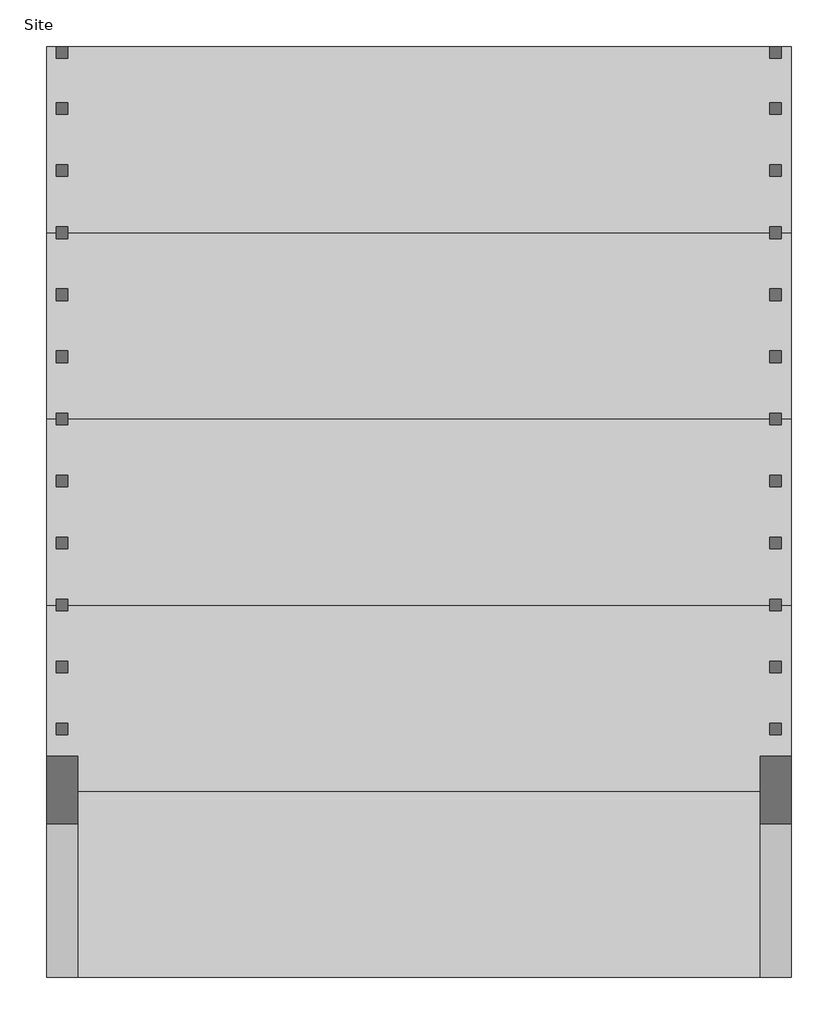
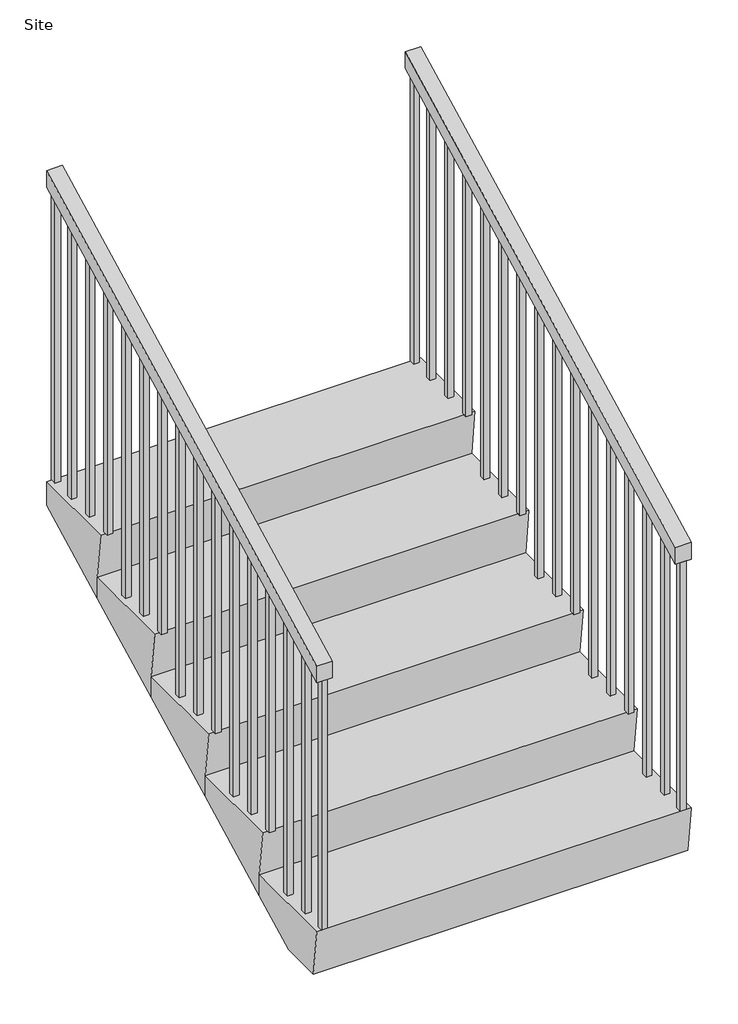
# One storey: 2 railings, 1 stair flight.
"""IFC4 building model written with IfcOpenShell, lengths in millimetres."""

from ifc_helpers import new_model, si_unit, frame, origin, place, context, project, spatial, polyline, outline, extrude, faceted_brep, element, save

model = new_model("IFC4")

# Units and contexts
model_context = context("Model", 3, world=origin())
ifc_project = project(units=[si_unit("LENGTHUNIT", "METRE", prefix="MILLI")], contexts=[model_context])

# Site, building, storey
site = spatial("IfcSite", under=ifc_project)
building = spatial("IfcBuilding", under=site)
storey = spatial("IfcBuildingStorey", under=building, Name="Site", Elevation=-939.8)

# Railings
placement = place(None, origin())
element("IfcRailing", 1, ObjectType="Handrail - Rectangular", at=placement, inside=storey, context=model_context, shape_type="SweptSolid", body=[
    extrude(outline(polyline([(-5687.1111242, 74.1181862), (-5687.1111242, 131.2333333), (-4163.1111242, 914.4), (-4163.1111242, 857.2848529), (-5687.1111242, 74.1181862)])), frame((-477.3803068, 0.0, 0.0), z_axis=(1.0, 0.0, 0.0), x_axis=(0.0, 1.0, 0.0)), (0.0, 0.0, 1.0), 50.8),
    extrude(outline(polyline([(-4274.2361242, 800.1789501), (-4255.1861242, 809.9685334), (-4255.1861242, -156.6333333), (-4274.2361242, -156.6333333), (-4274.2361242, 800.1789501)])), frame((-461.5053068, 0.0, 0.0), z_axis=(1.0, 0.0, 0.0), x_axis=(0.0, 1.0, 0.0)), (0.0, 0.0, 1.0), 19.05),
    extrude(outline(polyline([(-4375.8361242, 747.967839), (-4356.7861242, 757.7574223), (-4356.7861242, -156.6333333), (-4375.8361242, -156.6333333), (-4375.8361242, 747.967839)])), frame((-461.5053068, 0.0, 0.0), z_axis=(1.0, 0.0, 0.0), x_axis=(0.0, 1.0, 0.0)), (0.0, 0.0, 1.0), 19.05),
    extrude(outline(polyline([(-4477.4361242, 695.7567279), (-4458.3861242, 705.5463112), (-4458.3861242, -156.6333333), (-4477.4361242, -156.6333333), (-4477.4361242, 695.7567279)])), frame((-461.5053068, 0.0, 0.0), z_axis=(1.0, 0.0, 0.0), x_axis=(0.0, 1.0, 0.0)), (0.0, 0.0, 1.0), 19.05),
    extrude(outline(polyline([(-4579.0361242, 643.5456168), (-4559.9861242, 653.3352001), (-4559.9861242, -313.2666667), (-4579.0361242, -313.2666667), (-4579.0361242, 643.5456168)])), frame((-461.5053068, 0.0, 0.0), z_axis=(1.0, 0.0, 0.0), x_axis=(0.0, 1.0, 0.0)), (0.0, 0.0, 1.0), 19.05),
    extrude(outline(polyline([(-4680.6361242, 591.3345057), (-4661.5861242, 601.124089), (-4661.5861242, -313.2666667), (-4680.6361242, -313.2666667), (-4680.6361242, 591.3345057)])), frame((-461.5053068, 0.0, 0.0), z_axis=(1.0, 0.0, 0.0), x_axis=(0.0, 1.0, 0.0)), (0.0, 0.0, 1.0), 19.05),
    extrude(outline(polyline([(-4782.2361242, 539.1233945), (-4763.1861242, 548.9129779), (-4763.1861242, -313.2666667), (-4782.2361242, -313.2666667), (-4782.2361242, 539.1233945)])), frame((-461.5053068, 0.0, 0.0), z_axis=(1.0, 0.0, 0.0), x_axis=(0.0, 1.0, 0.0)), (0.0, 0.0, 1.0), 19.05),
    extrude(outline(polyline([(-4883.8361242, 486.9122834), (-4864.7861242, 496.7018668), (-4864.7861242, -469.9), (-4883.8361242, -469.9), (-4883.8361242, 486.9122834)])), frame((-461.5053068, 0.0, 0.0), z_axis=(1.0, 0.0, 0.0), x_axis=(0.0, 1.0, 0.0)), (0.0, 0.0, 1.0), 19.05),
    extrude(outline(polyline([(-4985.4361242, 434.7011723), (-4966.3861242, 444.4907557), (-4966.3861242, -469.9), (-4985.4361242, -469.9), (-4985.4361242, 434.7011723)])), frame((-461.5053068, 0.0, 0.0), z_axis=(1.0, 0.0, 0.0), x_axis=(0.0, 1.0, 0.0)), (0.0, 0.0, 1.0), 19.05),
    extrude(outline(polyline([(-5087.0361242, 382.4900612), (-5067.9861242, 392.2796445), (-5067.9861242, -469.9), (-5087.0361242, -469.9), (-5087.0361242, 382.4900612)])), frame((-461.5053068, 0.0, 0.0), z_axis=(1.0, 0.0, 0.0), x_axis=(0.0, 1.0, 0.0)), (0.0, 0.0, 1.0), 19.05),
    extrude(outline(polyline([(-5188.6361242, 330.2789501), (-5169.5861242, 340.0685334), (-5169.5861242, -626.5333333), (-5188.6361242, -626.5333333), (-5188.6361242, 330.2789501)])), frame((-461.5053068, 0.0, 0.0), z_axis=(1.0, 0.0, 0.0), x_axis=(0.0, 1.0, 0.0)), (0.0, 0.0, 1.0), 19.05),
    extrude(outline(polyline([(-5290.2361242, 278.067839), (-5271.1861242, 287.8574223), (-5271.1861242, -626.5333333), (-5290.2361242, -626.5333333), (-5290.2361242, 278.067839)])), frame((-461.5053068, 0.0, 0.0), z_axis=(1.0, 0.0, 0.0), x_axis=(0.0, 1.0, 0.0)), (0.0, 0.0, 1.0), 19.05),
    extrude(outline(polyline([(-5391.8361242, 225.8567279), (-5372.7861242, 235.6463112), (-5372.7861242, -626.5333333), (-5391.8361242, -626.5333333), (-5391.8361242, 225.8567279)])), frame((-461.5053068, 0.0, 0.0), z_axis=(1.0, 0.0, 0.0), x_axis=(0.0, 1.0, 0.0)), (0.0, 0.0, 1.0), 19.05),
    extrude(outline(polyline([(-5493.4361242, 173.6456168), (-5474.3861242, 183.4352001), (-5474.3861242, -783.1666667), (-5493.4361242, -783.1666667), (-5493.4361242, 173.6456168)])), frame((-461.5053068, 0.0, 0.0), z_axis=(1.0, 0.0, 0.0), x_axis=(0.0, 1.0, 0.0)), (0.0, 0.0, 1.0), 19.05),
    extrude(outline(polyline([(-5595.0361242, 121.4345057), (-5575.9861242, 131.224089), (-5575.9861242, -783.1666667), (-5595.0361242, -783.1666667), (-5595.0361242, 121.4345057)])), frame((-461.5053068, 0.0, 0.0), z_axis=(1.0, 0.0, 0.0), x_axis=(0.0, 1.0, 0.0)), (0.0, 0.0, 1.0), 19.05),
    extrude(outline(polyline([(-4182.1611242, 847.4952695), (-4163.1111242, 857.2848529), (-4163.1111242, -156.6333333), (-4182.1611242, -156.6333333), (-4182.1611242, 847.4952695)])), frame((-461.5053068, 0.0, 0.0), z_axis=(1.0, 0.0, 0.0), x_axis=(0.0, 1.0, 0.0)), (0.0, 0.0, 1.0), 19.05),
    extrude(outline(polyline([(-5687.1111242, 74.1181862), (-5668.0611242, 83.9077695), (-5668.0611242, -783.1666667), (-5687.1111242, -783.1666667), (-5687.1111242, 74.1181862)])), frame((-461.5053068, 0.0, 0.0), z_axis=(1.0, 0.0, 0.0), x_axis=(0.0, 1.0, 0.0)), (0.0, 0.0, 1.0), 19.05),
])
element("IfcRailing", 2, ObjectType="Handrail - Rectangular", at=placement, inside=storey, context=model_context, shape_type="SweptSolid", body=[
    extrude(outline(polyline([(-5687.1111242, 74.1181862), (-5687.1111242, 131.2333333), (-4163.1111242, 914.4), (-4163.1111242, 857.2848529), (-5687.1111242, 74.1181862)])), frame((-1645.7803068, 0.0, 0.0), z_axis=(1.0, 0.0, 0.0), x_axis=(0.0, 1.0, 0.0)), (0.0, 0.0, 1.0), 50.8),
    extrude(outline(polyline([(-4255.1861242, 809.9685334), (-4255.1861242, -156.6333333), (-4274.2361242, -156.6333333), (-4274.2361242, 800.1789501), (-4255.1861242, 809.9685334)])), frame((-1629.9053068, 0.0, 0.0), z_axis=(1.0, 0.0, 0.0), x_axis=(0.0, 1.0, 0.0)), (0.0, 0.0, 1.0), 19.05),
    extrude(outline(polyline([(-4356.7861242, 757.7574223), (-4356.7861242, -156.6333333), (-4375.8361242, -156.6333333), (-4375.8361242, 747.967839), (-4356.7861242, 757.7574223)])), frame((-1629.9053068, 0.0, 0.0), z_axis=(1.0, 0.0, 0.0), x_axis=(0.0, 1.0, 0.0)), (0.0, 0.0, 1.0), 19.05),
    extrude(outline(polyline([(-4458.3861242, 705.5463112), (-4458.3861242, -156.6333333), (-4477.4361242, -156.6333333), (-4477.4361242, 695.7567279), (-4458.3861242, 705.5463112)])), frame((-1629.9053068, 0.0, 0.0), z_axis=(1.0, 0.0, 0.0), x_axis=(0.0, 1.0, 0.0)), (0.0, 0.0, 1.0), 19.05),
    extrude(outline(polyline([(-4559.9861242, 653.3352001), (-4559.9861242, -313.2666667), (-4579.0361242, -313.2666667), (-4579.0361242, 643.5456168), (-4559.9861242, 653.3352001)])), frame((-1629.9053068, 0.0, 0.0), z_axis=(1.0, 0.0, 0.0), x_axis=(0.0, 1.0, 0.0)), (0.0, 0.0, 1.0), 19.05),
    extrude(outline(polyline([(-4661.5861242, 601.124089), (-4661.5861242, -313.2666667), (-4680.6361242, -313.2666667), (-4680.6361242, 591.3345057), (-4661.5861242, 601.124089)])), frame((-1629.9053068, 0.0, 0.0), z_axis=(1.0, 0.0, 0.0), x_axis=(0.0, 1.0, 0.0)), (0.0, 0.0, 1.0), 19.05),
    extrude(outline(polyline([(-4763.1861242, 548.9129779), (-4763.1861242, -313.2666667), (-4782.2361242, -313.2666667), (-4782.2361242, 539.1233945), (-4763.1861242, 548.9129779)])), frame((-1629.9053068, 0.0, 0.0), z_axis=(1.0, 0.0, 0.0), x_axis=(0.0, 1.0, 0.0)), (0.0, 0.0, 1.0), 19.05),
    extrude(outline(polyline([(-4864.7861242, 496.7018668), (-4864.7861242, -469.9), (-4883.8361242, -469.9), (-4883.8361242, 486.9122834), (-4864.7861242, 496.7018668)])), frame((-1629.9053068, 0.0, 0.0), z_axis=(1.0, 0.0, 0.0), x_axis=(0.0, 1.0, 0.0)), (0.0, 0.0, 1.0), 19.05),
    extrude(outline(polyline([(-4966.3861242, 444.4907557), (-4966.3861242, -469.9), (-4985.4361242, -469.9), (-4985.4361242, 434.7011723), (-4966.3861242, 444.4907557)])), frame((-1629.9053068, 0.0, 0.0), z_axis=(1.0, 0.0, 0.0), x_axis=(0.0, 1.0, 0.0)), (0.0, 0.0, 1.0), 19.05),
    extrude(outline(polyline([(-5067.9861242, 392.2796445), (-5067.9861242, -469.9), (-5087.0361242, -469.9), (-5087.0361242, 382.4900612), (-5067.9861242, 392.2796445)])), frame((-1629.9053068, 0.0, 0.0), z_axis=(1.0, 0.0, 0.0), x_axis=(0.0, 1.0, 0.0)), (0.0, 0.0, 1.0), 19.05),
    extrude(outline(polyline([(-5169.5861242, 340.0685334), (-5169.5861242, -626.5333333), (-5188.6361242, -626.5333333), (-5188.6361242, 330.2789501), (-5169.5861242, 340.0685334)])), frame((-1629.9053068, 0.0, 0.0), z_axis=(1.0, 0.0, 0.0), x_axis=(0.0, 1.0, 0.0)), (0.0, 0.0, 1.0), 19.05),
    extrude(outline(polyline([(-5271.1861242, 287.8574223), (-5271.1861242, -626.5333333), (-5290.2361242, -626.5333333), (-5290.2361242, 278.067839), (-5271.1861242, 287.8574223)])), frame((-1629.9053068, 0.0, 0.0), z_axis=(1.0, 0.0, 0.0), x_axis=(0.0, 1.0, 0.0)), (0.0, 0.0, 1.0), 19.05),
    extrude(outline(polyline([(-5372.7861242, 235.6463112), (-5372.7861242, -626.5333333), (-5391.8361242, -626.5333333), (-5391.8361242, 225.8567279), (-5372.7861242, 235.6463112)])), frame((-1629.9053068, 0.0, 0.0), z_axis=(1.0, 0.0, 0.0), x_axis=(0.0, 1.0, 0.0)), (0.0, 0.0, 1.0), 19.05),
    extrude(outline(polyline([(-5474.3861242, 183.4352001), (-5474.3861242, -783.1666667), (-5493.4361242, -783.1666667), (-5493.4361242, 173.6456168), (-5474.3861242, 183.4352001)])), frame((-1629.9053068, 0.0, 0.0), z_axis=(1.0, 0.0, 0.0), x_axis=(0.0, 1.0, 0.0)), (0.0, 0.0, 1.0), 19.05),
    extrude(outline(polyline([(-5575.9861242, 131.224089), (-5575.9861242, -783.1666667), (-5595.0361242, -783.1666667), (-5595.0361242, 121.4345057), (-5575.9861242, 131.224089)])), frame((-1629.9053068, 0.0, 0.0), z_axis=(1.0, 0.0, 0.0), x_axis=(0.0, 1.0, 0.0)), (0.0, 0.0, 1.0), 19.05),
    extrude(outline(polyline([(-4163.1111242, 857.2848529), (-4163.1111242, -156.6333333), (-4182.1611242, -156.6333333), (-4182.1611242, 847.4952695), (-4163.1111242, 857.2848529)])), frame((-1629.9053068, 0.0, 0.0), z_axis=(1.0, 0.0, 0.0), x_axis=(0.0, 1.0, 0.0)), (0.0, 0.0, 1.0), 19.05),
    extrude(outline(polyline([(-5668.0611242, 83.9077695), (-5668.0611242, -783.1666667), (-5687.1111242, -783.1666667), (-5687.1111242, 74.1181862), (-5668.0611242, 83.9077695)])), frame((-1629.9053068, 0.0, 0.0), z_axis=(1.0, 0.0, 0.0), x_axis=(0.0, 1.0, 0.0)), (0.0, 0.0, 1.0), 19.05),
])

# Stair flight
element("IfcStairFlight", 3, ObjectType="3/4\" Nosing", at=placement, inside=storey, context=model_context, shape_type="Brep", body=[
    faceted_brep([(-426.5803068, -5687.1111242, -783.1666667), (-1645.7803068, -5687.1111242, -783.1666667), (-1645.7803068, -5668.0611242, -939.8), (-426.5803068, -5668.0611242, -939.8), (-426.5803068, -5363.2611242, -783.1666667), (-1645.7803068, -5363.2611242, -783.1666667), (-1645.7803068, -5363.2611242, -854.5606006), (-1645.7803068, -5529.1323879, -939.8), (-426.5803068, -5529.1323879, -939.8), (-426.5803068, -5363.2611242, -854.5606006), (-1645.7803068, -5382.3111242, -626.5333333), (-426.5803068, -5382.3111242, -626.5333333), (-426.5803068, -5058.4611242, -626.5333333), (-1645.7803068, -5058.4611242, -626.5333333), (-1645.7803068, -5058.4611242, -697.9272672), (-426.5803068, -5058.4611242, -697.9272672), (-1645.7803068, -5077.5111242, -469.9), (-426.5803068, -5077.5111242, -469.9), (-426.5803068, -4753.6611242, -469.9), (-1645.7803068, -4753.6611242, -469.9), (-1645.7803068, -4753.6611242, -541.2939339), (-426.5803068, -4753.6611242, -541.2939339), (-1645.7803068, -4772.7111242, -313.2666667), (-426.5803068, -4772.7111242, -313.2666667), (-426.5803068, -4448.8611242, -313.2666667), (-1645.7803068, -4448.8611242, -313.2666667), (-1645.7803068, -4448.8611242, -384.6606006), (-426.5803068, -4448.8611242, -384.6606006), (-1645.7803068, -4467.9111242, -156.6333333), (-426.5803068, -4467.9111242, -156.6333333), (-426.5803068, -4163.1111242, -156.6333333), (-1645.7803068, -4163.1111242, -156.6333333), (-1645.7803068, -4163.1111242, -237.8168506), (-426.5803068, -4163.1111242, -237.8168506)], [[[0, 1, 2, 3]], [[1, 0, 4, 5]], [[1, 5, 6, 7, 2]], [[4, 0, 3, 8, 9]], [[10, 11, 12, 13]], [[10, 13, 14, 6, 5]], [[12, 11, 4, 9, 15]], [[5, 4, 11, 10]], [[16, 17, 18, 19]], [[16, 19, 20, 14, 13]], [[18, 17, 12, 15, 21]], [[13, 12, 17, 16]], [[22, 23, 24, 25]], [[22, 25, 26, 20, 19]], [[24, 23, 18, 21, 27]], [[19, 18, 23, 22]], [[28, 29, 30, 31]], [[28, 31, 32, 26, 25]], [[30, 29, 24, 27, 33]], [[31, 30, 33, 32]], [[25, 24, 29, 28]], [[3, 2, 7, 8]], [[8, 7, 6, 14, 20, 26, 32, 33, 27, 21, 15, 9]]]),
])

save(model, "model.ifc")

# Revit data of these elements
# Type "Handrail - Rectangular"
#   Assembly Code = "C2010400"
#   built-in parameter 1008612 = 0.0416667 (stored number, unit not read)
#   built-in parameter 1008611 = 0.0416667 (stored number, unit not read)
#   built-in parameter 1008609 = 0.333333 (stored number, unit not read)
#   built-in parameter 1008604 = 0.166667 (stored number, unit not read)
#   built-in parameter 1008603 = 0.166667 (stored number, unit not read)
#   Railing Height = 3' - 0"
#   built-in parameter 1008630 = 2
#   built-in parameter 1008610 = 2
#   built-in parameter 1008618 = Baluster - Square : 3/4"
# Elements 1, 2 (IfcRailing, "Handrail - Rectangular")
#   Phase Created = Existing
# Element 3 (IfcStairFlight, "3/4\" Nosing")
#   Phase Created = Existing
#   Materials on its faces: "Concrete, Cast-in-Place gray"
# Materials
#   "Concrete, Cast-in-Place gray": class "Concrete", colour RGB 192 192 192, transparency 0, Description = "Cast-in-place concrete", Cost = 0
